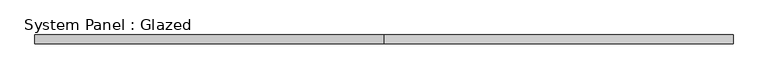
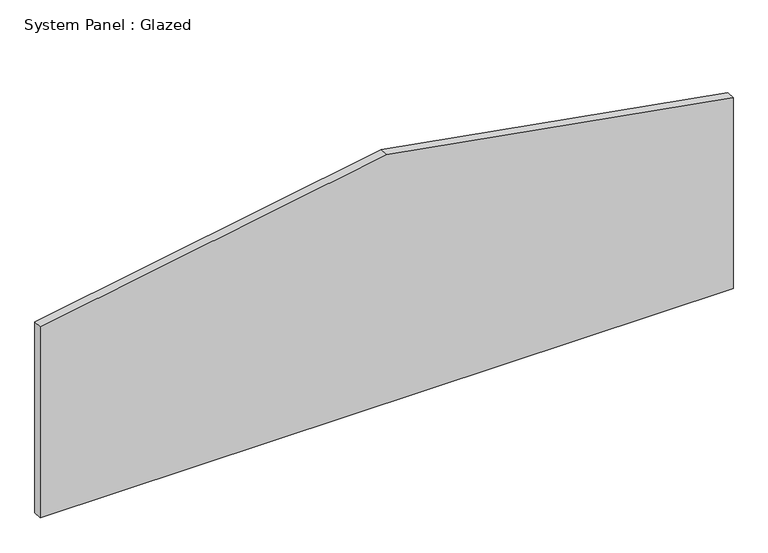
"""IFC4 building model written with IfcOpenShell, lengths in millimetres: plate geometry, System Panel : Glazed."""

from ifc_helpers import new_model, si_unit, frame, origin, place, context, project, spatial, polyline, outline, extrude, source, transform, mapped, element, save


def system_panel_glazed_0ee6ed81(model_context):
    return source(origin(), model_context, "Body", "SweptSolid", [
        extrude(outline(polyline([(0.0, -985.4757062), (0.0, 985.4757062), (574.4884442, 985.4757062), (748.2544, 0.0), (574.4884442, -985.4757062), (0.0, -985.4757062)])), frame((0.0, -44.45, 0.0), z_axis=(0.0, 1.0, 0.0), x_axis=(0.0, 0.0, 1.0)), (0.0, 0.0, 1.0), 25.4),
    ])


if __name__ == "__main__":
    model = new_model("IFC4")
    model_context = context("Model", 3, world=origin())
    ifc_project = project(units=[si_unit("LENGTHUNIT", "METRE", prefix="MILLI")], contexts=[model_context])
    site = spatial("IfcSite", under=ifc_project)
    building = spatial("IfcBuilding", under=site)
    placement = place(None, origin())
    system_panel_glazed_shape = system_panel_glazed_0ee6ed81(model_context)
    element("IfcPlate", 1, ObjectType="System Panel : Glazed", at=placement, inside=building, context=model_context, shape_type="MappedRepresentation", body=[
        mapped(system_panel_glazed_shape, transform((0.0, 0.0, 0.0), x_axis=(1.0, 0.0, 0.0), y_axis=(0.0, 1.0, 0.0), z_axis=(0.0, 0.0, 1.0))),
    ])
    save(model, "model.ifc")

# Revit data of these elements
# Element 1 (IfcPlate, "System Panel : Glazed")
#   Materials on its faces: "Glass"
# Materials
#   "Glass": class "Unassigned", colour RGB 147 173 200, transparency 0.7, Cost = 0
